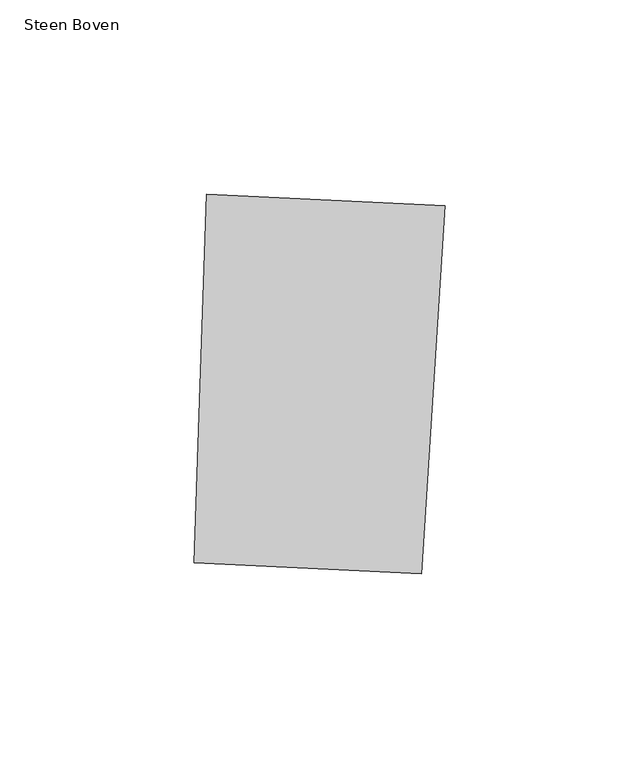
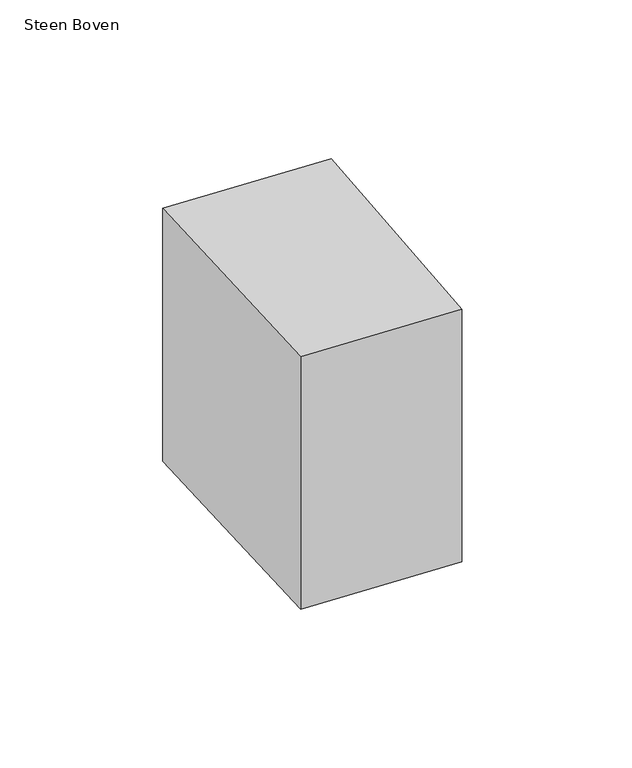
"""IFC4 building model written with IfcOpenShell, lengths in millimetres: proxy geometry, 00_GMA_steen_versie_4 : Steen Boven."""

from ifc_helpers import new_model, si_unit, origin, origin_with_axes, place, context, project, spatial, polyline, outline, extrude, source, transform, mapped, element, save


def steen_boven_8e64520f(model_context):
    return source(origin(), model_context, "Body", "SweptSolid", [
        extrude(outline(polyline([(103.7126267, 118.7458736), (97.720871, 23.9247913), (39.0765598, 26.7901699), (42.3572493, 121.7437157), (103.7126267, 118.7458736)])), origin_with_axes(), (0.0, 0.0, 1.0), 100.0),
    ])


if __name__ == "__main__":
    model = new_model("IFC4")
    model_context = context("Model", 3, world=origin())
    ifc_project = project(units=[si_unit("LENGTHUNIT", "METRE", prefix="MILLI")], contexts=[model_context])
    site = spatial("IfcSite", under=ifc_project)
    building = spatial("IfcBuilding", under=site)
    placement = place(None, origin())
    steen_boven_shape = steen_boven_8e64520f(model_context)
    element("IfcBuildingElementProxy", 1, Name="00_GMA_steen_versie_4 : Steen Boven", ObjectType="00_GMA_steen_versie_4 : Steen Boven", at=placement, inside=building, context=model_context, shape_type="MappedRepresentation", body=[
        mapped(steen_boven_shape, transform((0.0, 0.0, 0.0), x_axis=(1.0, 0.0, 0.0), y_axis=(0.0, 1.0, 0.0), z_axis=(0.0, 0.0, 1.0))),
    ])
    save(model, "model.ifc")

# Revit data of these elements
# Type "00_GMA_steen_versie_4 : Steen Boven"
#   StootVoegHalfBoven [instance default] = 5 mm
#   StootVoegHalf [instance default] = 5 mm
#   StootVoegBreedteOnder = 10 mm
#   StootVoegBreedteBoven = 10 mm
#   Steendikte = 100 mm
#   LintVoegOnderHalf = 5 mm
#   LintVoegOnder = 10 mm
#   LintVoegBovenHalf = 0 mm
#   LintVoegBoven = 0 mm
#   materiaal = none
#   MateriaalVoeg = none
#   Default Elevation = 0
